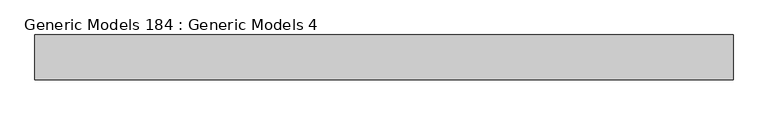
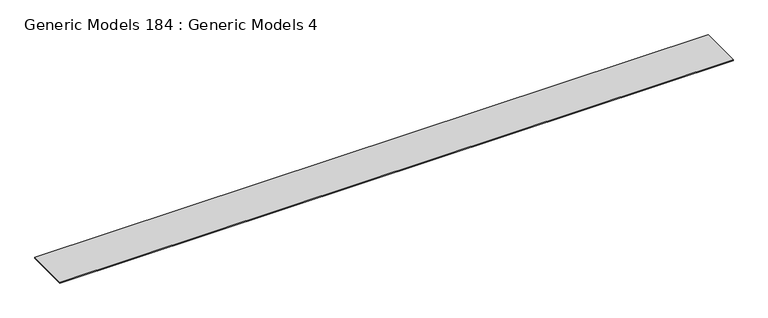
"""IFC4 building model written with IfcOpenShell, lengths in millimetres: proxy geometry, Generic Models 184 : Generic Models 4."""

import ifcopenshell
import ifcopenshell.guid

model = None  # the IFC model being written
_history = None  # IfcOwnerHistory: only IFC2X3 demands one
_inside = {}  # id of a spatial element -> (the spatial element, [elements in it])
_under = {}  # id of a project, library or spatial element -> (it, [spatial elements below it])
_declared = {}  # id of a project -> (the project, [libraries it declares])
_typed = {}  # id of a type object -> (the type object, [elements of that type])
_made_of = {}  # id of a material, layer set ... -> (it, [elements and type objects made of it])


def new_model(schema):
    """Start an empty IFC model of exactly this schema.

    Asked for "IFC4X3", IfcOpenShell would pick the latest addendum, in which some entities
    have other attributes; the version numbers below select the first issue.
    IFC2X3 requires an IfcOwnerHistory on every rooted entity: one is made here for all.
    """
    global model, _history
    if schema == "IFC4X3":
        model = ifcopenshell.file(schema_version=(4, 3, 0, 0))
    else:
        model = ifcopenshell.file(schema=schema)
    _inside.clear()
    _under.clear()
    _declared.clear()
    _typed.clear()
    _made_of.clear()
    _history = None
    if model.schema == "IFC2X3":
        org = make("IfcOrganization", Name="unknown")
        user = make(
            "IfcPersonAndOrganization",
            ThePerson=make("IfcPerson", FamilyName="unknown"),
            TheOrganization=org,
        )
        app = make(
            "IfcApplication",
            ApplicationDeveloper=org,
            Version="unknown",
            ApplicationFullName="unknown",
            ApplicationIdentifier="unknown",
        )
        _history = make(
            "IfcOwnerHistory",
            OwningUser=user,
            OwningApplication=app,
            ChangeAction="ADDED",
            CreationDate=0,
        )
    return model


def make(cls, **values):
    """One entity of the class cls with the attributes given. An attribute that is None is left unset."""
    return model.create_entity(
        cls, **{name: value for name, value in values.items() if value is not None}
    )


def rooted(cls, **values):
    """An entity with a GlobalId (a new one), such as an element, a storey or a relation."""
    return make(cls, GlobalId=ifcopenshell.guid.new(), OwnerHistory=_history, **values)


def si_unit(unit_type, name, prefix=None):
    """IfcSIUnit, for example si_unit("LENGTHUNIT", "METRE", prefix="MILLI")."""
    return make("IfcSIUnit", UnitType=unit_type, Prefix=prefix, Name=name)


def assignment(units):
    """IfcUnitAssignment: the units of a project."""
    return None if units is None else make("IfcUnitAssignment", Units=units)


def point(xyz):
    """IfcCartesianPoint."""
    return None if xyz is None else make("IfcCartesianPoint", Coordinates=xyz)


def direction(xyz):
    """IfcDirection."""
    return None if xyz is None else make("IfcDirection", DirectionRatios=xyz)


def frame(location, z_axis=None, x_axis=None):
    """IfcAxis2Placement3D, a coordinate frame: its origin and axes. An axis left out is left unset."""
    return make(
        "IfcAxis2Placement3D",
        Location=point(location),
        Axis=direction(z_axis),
        RefDirection=direction(x_axis),
    )


def origin():
    """The frame at (0, 0, 0) with its axes left unset."""
    return frame((0.0, 0.0, 0.0))


def place(relative_to, where):
    """IfcLocalPlacement: puts the frame where relative to a parent placement (None: the world)."""
    return make(
        "IfcLocalPlacement", PlacementRelTo=relative_to, RelativePlacement=where
    )


def context(
    kind, dimensions, precision=None, world=None, true_north=None, identifier=None
):
    """IfcGeometricRepresentationContext, for example the 3D "Model" context."""
    return make(
        "IfcGeometricRepresentationContext",
        ContextIdentifier=identifier,
        ContextType=kind,
        CoordinateSpaceDimension=dimensions,
        Precision=precision,
        WorldCoordinateSystem=world,
        TrueNorth=true_north,
    )


def project(units=None, contexts=None):
    """IfcProject with its units and contexts."""
    return rooted(
        "IfcProject",
        Name="project",
        RepresentationContexts=contexts,
        UnitsInContext=assignment(units),
    )


def spatial(cls, under=None, at=None, **own):
    """A site, building, storey or space (cls), placed at a placement, below another one or the project."""
    s = rooted(cls, ObjectPlacement=at, **own)
    if under is not None:
        _under.setdefault(under.id(), (under, []))[1].append(s)
    return s


def polyline(points):
    """IfcPolyline through the points."""
    return make("IfcPolyline", Points=[point(p) for p in points])


def outline(outer, holes=None, kind="AREA"):
    """IfcArbitraryClosedProfileDef: a profile drawn as a closed curve; with holes, ...WithVoids."""
    if holes is None:
        return make("IfcArbitraryClosedProfileDef", ProfileType=kind, OuterCurve=outer)
    return make(
        "IfcArbitraryProfileDefWithVoids",
        ProfileType=kind,
        OuterCurve=outer,
        InnerCurves=holes,
    )


def extrude(swept, where, along, depth):
    """IfcExtrudedAreaSolid: the profile swept, set in the frame where, extruded along a direction by depth."""
    return make(
        "IfcExtrudedAreaSolid",
        SweptArea=swept,
        Position=where,
        ExtrudedDirection=direction(along),
        Depth=depth,
    )


def shape(context_of_items, identifier, shape_type, items):
    """IfcShapeRepresentation: the items that make up one representation, for example the "Body"."""
    return make(
        "IfcShapeRepresentation",
        ContextOfItems=context_of_items,
        RepresentationIdentifier=identifier,
        RepresentationType=shape_type,
        Items=items,
    )


def source(mapping_origin, context_of_items, identifier, shape_type, items):
    """IfcRepresentationMap: a shape defined once, which mapped items show again and again."""
    return make(
        "IfcRepresentationMap",
        MappingOrigin=mapping_origin,
        MappedRepresentation=shape(context_of_items, identifier, shape_type, items),
    )


def transform(
    local_origin,
    x_axis=None,
    y_axis=None,
    z_axis=None,
    scale=None,
    scale2=None,
    scale3=None,
    uniform=True,
):
    """IfcCartesianTransformationOperator3D, or its non-uniform kind. x_axis, y_axis, z_axis: its Axis1, 2, 3."""
    if uniform:
        return make(
            "IfcCartesianTransformationOperator3D",
            Axis1=direction(x_axis),
            Axis2=direction(y_axis),
            LocalOrigin=point(local_origin),
            Scale=scale,
            Axis3=direction(z_axis),
        )
    return make(
        "IfcCartesianTransformationOperator3DnonUniform",
        Axis1=direction(x_axis),
        Axis2=direction(y_axis),
        LocalOrigin=point(local_origin),
        Scale=scale,
        Axis3=direction(z_axis),
        Scale2=scale2,
        Scale3=scale3,
    )


def mapped(mapping_source, mapping_target):
    """IfcMappedItem: shows the shape of a source again, moved by a transform."""
    return make(
        "IfcMappedItem", MappingSource=mapping_source, MappingTarget=mapping_target
    )


def made_of(thing, what):
    """Note that an element or type object is made of a material, layer set ...; save() writes the relation."""
    if what is not None:
        _made_of.setdefault(what.id(), (what, []))[1].append(thing)
    return thing


def element(
    cls,
    number,
    at=None,
    inside=None,
    cuts=None,
    type_object=None,
    material=None,
    context=None,
    identifier="Body",
    shape_type=None,
    held_by="IfcProductDefinitionShape",
    body=None,
    shapes=None,
    **own,
):
    """One element of the class cls, such as IfcWall. Its Tag is "e" and its number.

    at: its placement. inside: the storey or other place that contains it. cuts: it is an
    opening in that element (IfcRelVoidsElement). A single representation is given by context,
    identifier, shape_type and body (its items); several are given by shapes. held_by: the class
    of the entity that holds the representations. save() writes the other relations.
    """
    e = rooted(cls, Tag="e%d" % number, ObjectPlacement=at, **own)
    if body is not None:
        shapes = [shape(context, identifier, shape_type, body)]
    if shapes is not None:
        e.Representation = make(held_by, Representations=shapes)
    if inside is not None:
        _inside.setdefault(inside.id(), (inside, []))[1].append(e)
    if cuts is not None:
        rooted(
            "IfcRelVoidsElement", RelatingBuildingElement=cuts, RelatedOpeningElement=e
        )
    if type_object is not None:
        _typed.setdefault(type_object.id(), (type_object, []))[1].append(e)
    return made_of(e, material)


def aggregate(whole, parts):
    """IfcRelAggregates: a whole, such as a stair, and the parts it consists of."""
    return rooted("IfcRelAggregates", RelatingObject=whole, RelatedObjects=parts)


def save(model, path):
    """Write the relations noted so far, then the file.

    IfcRelAggregates (storeys below a building ...), IfcRelContainedInSpatialStructure (elements
    in a storey), IfcRelDefinesByType, IfcRelAssociatesMaterial and IfcRelDeclares: one each for
    every whole, place, type object, material and project.
    """
    for whole, parts in _under.values():
        aggregate(whole, parts)
    for where, things in _inside.values():
        rooted(
            "IfcRelContainedInSpatialStructure",
            RelatedElements=things,
            RelatingStructure=where,
        )
    for kind, things in _typed.values():
        rooted("IfcRelDefinesByType", RelatedObjects=things, RelatingType=kind)
    for what, things in _made_of.values():
        rooted("IfcRelAssociatesMaterial", RelatedObjects=things, RelatingMaterial=what)
    for by, libraries in _declared.values():
        rooted("IfcRelDeclares", RelatingContext=by, RelatedDefinitions=libraries)
    model.write(path)


def generic_models_184_generic_models_4_fb8d16b8(model_context):
    return source(origin(), model_context, "Body", "SweptSolid", [
        extrude(outline(polyline([(2196.9263704, -6080.7311742), (2196.9263704, -6871.9053756), (-10098.8420874, -6871.9053756), (-10098.8420874, -6080.7311742), (2196.9263704, -6080.7311742)])), frame((0.0, 0.0, 126355.8662959), z_axis=(0.0, 0.0, 1.0), x_axis=(1.0, 0.0, 0.0)), (0.0, 0.0, 1.0), 15.875),
    ])


if __name__ == "__main__":
    model = new_model("IFC4")
    model_context = context("Model", 3, world=origin())
    ifc_project = project(units=[si_unit("LENGTHUNIT", "METRE", prefix="MILLI")], contexts=[model_context])
    site = spatial("IfcSite", under=ifc_project)
    building = spatial("IfcBuilding", under=site)
    placement = place(None, origin())
    generic_models_184_generic_models_4_shape = generic_models_184_generic_models_4_fb8d16b8(model_context)
    element("IfcBuildingElementProxy", 1, Name="Generic Models 184 : Generic Models 4", ObjectType="Generic Models 184 : Generic Models 4", at=placement, inside=building, context=model_context, shape_type="MappedRepresentation", body=[
        mapped(generic_models_184_generic_models_4_shape, transform((0.0, 0.0, 0.0), x_axis=(1.0, 0.0, 0.0), y_axis=(0.0, 1.0, 0.0), z_axis=(0.0, 0.0, 1.0))),
    ])
    save(model, "model.ifc")

# Revit data of these elements
# Element 1 (IfcBuildingElementProxy, "Generic Models 184 : Generic Models 4")
#   Materials on its faces: "_5/8\" DRYWALL"
# Materials
#   "_5/8\" DRYWALL": class "Generic", colour RGB 191 191 191, transparency 0, Cost = 0
